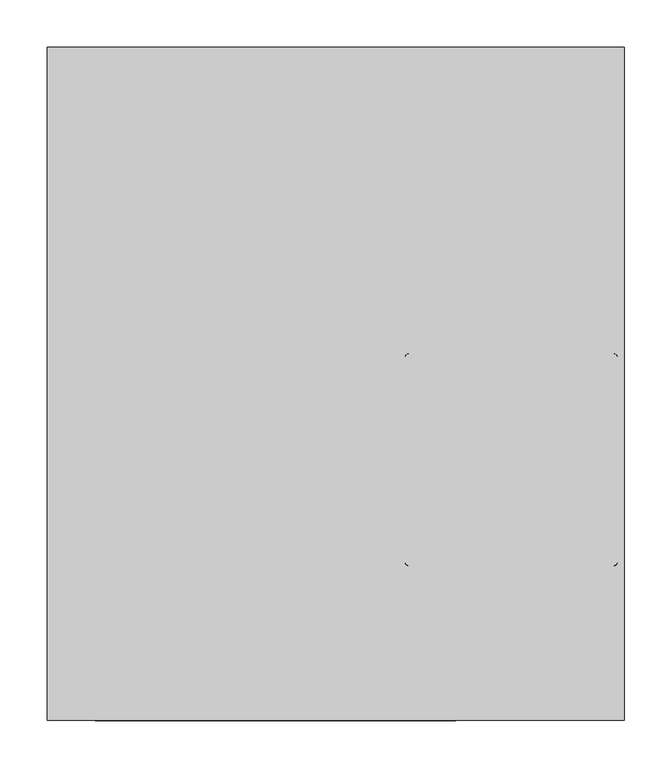
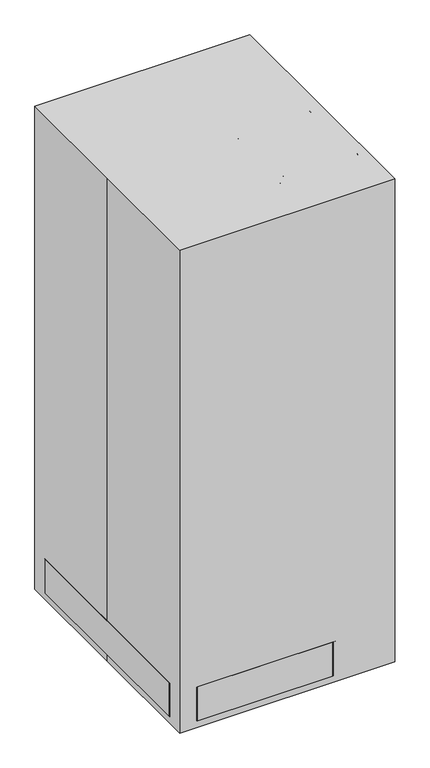
"""IFC4 building model written with IfcOpenShell, lengths in millimetres: proxy geometry, M1715 - Hemodialysis Unit, Hollow Fiber or Plate : M1715 - Hemodialysis Unit, Hollow Fiber or Plate."""

from ifc_helpers import new_model, si_unit, point, frame, frame_2d, origin, origin_with_axes, place, context, project, spatial, polyline, circle_curve, ellipse_curve, trimmed, segment, composite_curve, outline, extrude, source, transform, mapped, element, save
from ifc_brep_helpers import plane_surface, cylinder_surface, revolved_surface, advanced_brep


def specialty_equipment_02c0782f(model_context):
    return source(origin(), model_context, "Body", "SolidModel", [
        extrude(outline(polyline([(12.8462109, 171.45), (12.8462109, 165.1), (-152.2537891, 165.1), (-152.2537891, 171.45), (12.8462109, 171.45)])), frame((0.0, 0.0, 953.8161521), z_axis=(0.0, 0.0, 1.0), x_axis=(1.0, 0.0, 0.0)), (0.0, 0.0, 1.0), 127.0),
        extrude(outline(polyline([(152.4, -101.6), (209.55, -101.6), (209.55, -55.2125267), (152.4, -55.2125267), (152.4, -42.5125267), (222.25, -42.5125267), (222.25, -114.3), (152.4, -114.3), (152.4, -101.6)])), frame((0.0, 0.0, 812.8), z_axis=(0.0, 0.0, 1.0), x_axis=(1.0, 0.0, 0.0)), (0.0, 0.0, 1.0), 25.4),
        extrude(outline(polyline([(928.4161521, 38.2462109), (1106.2161521, 38.2462109), (1106.2161521, -177.6537891), (928.4161521, -177.6537891), (928.4161521, 38.2462109)]), holes=[polyline([(1080.8161521, -152.2537891), (1080.8161521, 12.8462109), (953.8161521, 12.8462109), (953.8161521, -152.2537891), (1080.8161521, -152.2537891)])]), frame((0.0, 165.1, 0.0), z_axis=(0.0, 1.0, 0.0), x_axis=(0.0, 0.0, 1.0)), (0.0, 0.0, 1.0), 6.35),
        extrude(outline(polyline([(421.0082083, 215.9), (421.0082083, 152.4), (281.3082083, 152.4), (344.8082083, 215.9), (421.0082083, 215.9)])), frame((0.0, -117.475, 0.0), z_axis=(0.0, 1.0, 0.0), x_axis=(0.0, 0.0, 1.0)), (0.0, 0.0, 1.0), 76.2),
        extrude(outline(composite_curve([segment(trimmed(circle_curve(frame_2d((555.4484832, 75.5254157)), 19.05), [point((555.4484832, 56.4754157))], [point((555.4484832, 94.5754157))], False, "CARTESIAN"), True, "CONTINUOUS"), segment(trimmed(circle_curve(frame_2d((555.4484832, 75.5254157)), 19.05), [point((555.4484832, 94.5754157))], [point((555.4484832, 56.4754157))], False, "CARTESIAN"), True, "CONTINUOUS")], self_intersect=False)), frame((0.0, 165.1, 0.0), z_axis=(0.0, 1.0, 0.0), x_axis=(0.0, 0.0, 1.0)), (0.0, 0.0, 1.0), 38.1),
        extrude(outline(composite_curve([segment(trimmed(circle_curve(frame_2d((555.4484832, 15.2004157)), 19.05), [point((555.4484832, -3.8495843))], [point((555.4484832, 34.2504157))], False, "CARTESIAN"), True, "CONTINUOUS"), segment(trimmed(circle_curve(frame_2d((555.4484832, 15.2004157)), 19.05), [point((555.4484832, 34.2504157))], [point((555.4484832, -3.8495843))], False, "CARTESIAN"), True, "CONTINUOUS")], self_intersect=False)), frame((0.0, 165.1, 0.0), z_axis=(0.0, 1.0, 0.0), x_axis=(0.0, 0.0, 1.0)), (0.0, 0.0, 1.0), 38.1),
        extrude(outline(composite_curve([segment(trimmed(circle_curve(frame_2d((555.4484832, -48.2995843)), 19.05), [point((555.4484832, -67.3495843))], [point((555.4484832, -29.2495843))], False, "CARTESIAN"), True, "CONTINUOUS"), segment(trimmed(circle_curve(frame_2d((555.4484832, -48.2995843)), 19.05), [point((555.4484832, -29.2495843))], [point((555.4484832, -67.3495843))], False, "CARTESIAN"), True, "CONTINUOUS")], self_intersect=False)), frame((0.0, 165.1, 0.0), z_axis=(0.0, 1.0, 0.0), x_axis=(0.0, 0.0, 1.0)), (0.0, 0.0, 1.0), 38.1),
        extrude(outline(composite_curve([segment(trimmed(circle_curve(frame_2d((555.4470563, -115.3669113)), 19.05), [point((555.4470563, -134.4169113))], [point((555.4470563, -96.3169113))], False, "CARTESIAN"), True, "CONTINUOUS"), segment(trimmed(circle_curve(frame_2d((555.4470563, -115.3669113)), 19.05), [point((555.4470563, -96.3169113))], [point((555.4470563, -134.4169113))], False, "CARTESIAN"), True, "CONTINUOUS")], self_intersect=False)), frame((0.0, 165.1, 0.0), z_axis=(0.0, 1.0, 0.0), x_axis=(0.0, 0.0, 1.0)), (0.0, 0.0, 1.0), 38.1),
        extrude(outline(polyline([(136.6593258, 165.1), (136.6593258, 127.0), (60.4593258, 127.0), (60.4593258, 165.1), (136.6593258, 165.1)])), frame((0.0, 0.0, 792.3608314), z_axis=(0.0, 0.0, 1.0), x_axis=(1.0, 0.0, 0.0)), (0.0, 0.0, 1.0), 38.1),
        extrude(outline(polyline([(36.523558, 165.1), (36.523558, 127.0), (-39.676442, 127.0), (-39.676442, 165.1), (36.523558, 165.1)])), frame((0.0, 0.0, 716.1608314), z_axis=(0.0, 0.0, 1.0), x_axis=(1.0, 0.0, 0.0)), (0.0, 0.0, 1.0), 114.3),
        extrude(outline(polyline([(-66.5406742, 165.1), (-66.5406742, 127.0), (-142.7406742, 127.0), (-142.7406742, 165.1), (-66.5406742, 165.1)])), frame((0.0, 0.0, 716.1608314), z_axis=(0.0, 0.0, 1.0), x_axis=(1.0, 0.0, 0.0)), (0.0, 0.0, 1.0), 114.3),
        extrude(outline(polyline([(-180.8406742, 165.1), (-180.8406742, 127.0), (-257.0406742, 127.0), (-257.0406742, 165.1), (-180.8406742, 165.1)])), frame((0.0, 0.0, 716.1608314), z_axis=(0.0, 0.0, 1.0), x_axis=(1.0, 0.0, 0.0)), (0.0, 0.0, 1.0), 38.1),
        extrude(outline(polyline([(-180.8406742, 165.1), (-180.8406742, 127.0), (-257.0406742, 127.0), (-257.0406742, 165.1), (-180.8406742, 165.1)])), frame((0.0, 0.0, 792.3608314), z_axis=(0.0, 0.0, 1.0), x_axis=(1.0, 0.0, 0.0)), (0.0, 0.0, 1.0), 38.1),
        extrude(outline(polyline([(140.5982906, 165.1), (140.5982906, 127.0), (-265.8017094, 127.0), (-265.8017094, 165.1), (140.5982906, 165.1)])), frame((0.0, 0.0, 446.4082083), z_axis=(0.0, 0.0, 1.0), x_axis=(1.0, 0.0, 0.0)), (0.0, 0.0, 1.0), 219.3819435),
        extrude(outline(polyline([(140.5982906, 165.1), (140.5982906, 127.0), (-265.8017094, 127.0), (-265.8017094, 165.1), (140.5982906, 165.1)])), frame((0.0, 0.0, 903.6082083), z_axis=(0.0, 0.0, 1.0), x_axis=(1.0, 0.0, 0.0)), (0.0, 0.0, 1.0), 219.3819435),
        extrude(outline(polyline([(140.5982906, 165.1), (140.5982906, 127.0), (-265.8017094, 127.0), (-265.8017094, 165.1), (140.5982906, 165.1)])), frame((0.0, 0.0, 132.3901517), z_axis=(0.0, 0.0, 1.0), x_axis=(1.0, 0.0, 0.0)), (0.0, 0.0, 1.0), 304.8),
        extrude(outline(polyline([(152.4, 127.0), (152.4, -279.4), (-279.4, -279.4), (-279.4, 127.0), (152.4, 127.0)])), frame((0.0, 0.0, 120.65), z_axis=(0.0, 0.0, 1.0), x_axis=(1.0, 0.0, 0.0)), (0.0, 0.0, 1.0), 1016.0),
        extrude(outline(composite_curve([segment(trimmed(circle_curve(frame_2d((185.3788167, -80.0577972)), 6.35), [point((179.0288167, -80.0577972))], [point((191.7288167, -80.0577972))], False, "CARTESIAN"), True, "CONTINUOUS"), segment(trimmed(circle_curve(frame_2d((185.3788167, -80.0577972)), 6.35), [point((191.7288167, -80.0577972))], [point((179.0288167, -80.0577972))], False, "CARTESIAN"), True, "CONTINUOUS")], self_intersect=False)), frame((0.0, 0.0, 1041.4), z_axis=(0.0, 0.0, 1.0), x_axis=(1.0, 0.0, 0.0)), (0.0, 0.0, 1.0), 388.3436057),
        advanced_brep(
        [(268.446484, -163.1254645, 1421.2516191), (264.5038206, -159.1828011, 1413.5291561), (276.9334178, -171.6123983, 1400.8374235), (280.8760812, -175.5550617, 1408.5598865), (284.1616341, -178.8406146, 1432.4577724), (284.1616341, -178.8406146, 1422.9327724), (86.5959994, 18.7250201, 1432.4577724), (86.5959994, 18.7250201, 1422.9327724), (93.8242157, 11.4968038, 1400.8374235), (89.8815523, 15.4394673, 1408.5598865), (102.3111494, 3.0098701, 1421.2516191), (106.2538129, -0.9327933, 1413.5291561)],
        [
            (0, 1, circle_curve(frame((266.4751523, -161.1541328, 1417.3903876), z_axis=(-0.5732919666883985, 0.5732919666884023, 0.5853824748496423), x_axis=(-0.41392791755394504, 0.41392791755394626, -0.8107572744902805)), 4.7625)),
            (1, 0, circle_curve(frame((266.4751523, -161.1541328, 1417.3903876), z_axis=(-0.5732919666883985, 0.5732919666884023, 0.5853824748496423), x_axis=(-0.41392791755394504, 0.41392791755394626, -0.8107572744902805)), 4.7625)),
            (1, 2),
            (2, 3, circle_curve(frame((278.9047495, -173.58373, 1404.698655), z_axis=(-0.5732919666883985, 0.5732919666884023, 0.5853824748496423), x_axis=(-0.41392791755394504, 0.41392791755394626, -0.8107572744902805)), 4.7625)),
            (3, 0),
            (3, 2, circle_curve(frame((278.9047495, -173.58373, 1404.698655), z_axis=(-0.5732919666883985, 0.5732919666884023, 0.5853824748496423), x_axis=(-0.41392791755394504, 0.41392791755394626, -0.8107572744902805)), 4.7625)),
            (4, 5, circle_curve(frame((284.1616341, -178.8406146, 1427.6952724), z_axis=(0.7071067811865466, -0.7071067811865487, 0.0), x_axis=(0.0, 0.0, 1.0)), 4.7625)),
            (5, 3, circle_curve(frame((284.1616341, -178.8406146, 1414.9952724), z_axis=(0.7071067811865489, 0.7071067811865462, 0.0), x_axis=(-0.413927917553943, 0.4139279175539444, -0.8107572744902825)), 7.9375)),
            (2, 4, circle_curve(frame((284.1616341, -178.8406146, 1414.9952724), z_axis=(-0.7071067811865489, -0.7071067811865462, 0.0), x_axis=(-0.413927917553943, 0.4139279175539444, -0.8107572744902825)), 17.4625)),
            (5, 4, circle_curve(frame((284.1616341, -178.8406146, 1427.6952724), z_axis=(0.7071067811865465, -0.7071067811865486, 0.0), x_axis=(0.0, 0.0, 1.0)), 4.7625)),
            (4, 6),
            (6, 7, circle_curve(frame((86.5959994, 18.7250201, 1427.6952724), z_axis=(0.7071067811865464, -0.7071067811865488, 0.0), x_axis=(0.0, 0.0, 1.0)), 4.7625)),
            (7, 5),
            (7, 6, circle_curve(frame((86.5959994, 18.7250201, 1427.6952724), z_axis=(0.7071067811865464, -0.7071067811865488, 0.0), x_axis=(0.0, 0.0, 1.0)), 4.7625)),
            (8, 9, circle_curve(frame((91.852884, 13.4681356, 1404.698655), z_axis=(-0.5732919666879008, 0.5732919666879034, -0.5853824748506183), x_axis=(0.4139279175546348, -0.41392791755463687, -0.8107572744895757)), 4.7625)),
            (9, 7, circle_curve(frame((86.5959994, 18.7250201, 1414.9952724), z_axis=(0.7071067811865489, 0.7071067811865462, 0.0), x_axis=(0.0, 0.0, 1.0)), 7.9375)),
            (6, 8, circle_curve(frame((86.5959994, 18.7250201, 1414.9952724), z_axis=(-0.7071067811865489, -0.7071067811865462, 0.0), x_axis=(0.0, 0.0, 1.0)), 17.4625)),
            (9, 8, circle_curve(frame((91.852884, 13.4681356, 1404.698655), z_axis=(-0.5732919666886381, 0.5732919666886407, -0.5853824748491742), x_axis=(0.41392791755361363, -0.4139279175536157, -0.8107572744906184)), 4.7625)),
            (10, 11, circle_curve(frame((104.2824812, 1.0385384, 1417.3903876), z_axis=(0.5732919666881265, -0.57329196668813, 0.5853824748501754), x_axis=(0.4139279175543215, -0.4139279175543237, -0.8107572744898957)), 4.7625)),
            (11, 10, circle_curve(frame((104.2824812, 1.0385384, 1417.3903876), z_axis=(0.5732919666881265, -0.57329196668813, 0.5853824748501754), x_axis=(0.4139279175543215, -0.4139279175543237, -0.8107572744898957)), 4.7625)),
            (8, 11),
            (10, 9),
        ],
        [
            plane_surface(frame((455.0605309, 27.4312457, 1417.3903876), z_axis=(-0.5732919666883985, 0.5732919666884023, 0.5853824748496423), x_axis=(-0.7071067811865496, -0.7071067811865456, 0.0))),
            cylinder_surface(frame((266.4751523, -161.1541328, 1417.3903876), z_axis=(-0.5732919666883985, 0.5732919666884023, 0.5853824748496423), x_axis=(-0.41392791755394504, 0.41392791755394626, -0.8107572744902805)), 4.7625),
            revolved_surface(trimmed(ellipse_curve(frame((278.9047495, -173.58373, 1404.698655), z_axis=(0.5732919666884007, -0.5732919666884032, -0.5853824748496393), x_axis=(-0.4139279175539432, 0.413927917553944, -0.8107572744902826)), 4.7625, 4.7625), [point((280.8760812, -175.5550617, 1408.5598865))], [point((276.9334178, -171.6123983, 1400.8374235))], True, "CARTESIAN"), (472.7470126, 9.744764, 1414.9952724), (0.7071067811865489, 0.7071067811865462, 0.0)),
            revolved_surface(trimmed(ellipse_curve(frame((278.9047495, -173.58373, 1404.698655), z_axis=(0.5732919666884007, -0.5732919666884032, -0.5853824748496393), x_axis=(-0.4139279175539432, 0.413927917553944, -0.8107572744902826)), 4.7625, 4.7625), [point((276.9334178, -171.6123983, 1400.8374235))], [point((280.8760812, -175.5550617, 1408.5598865))], True, "CARTESIAN"), (472.7470126, 9.744764, 1414.9952724), (0.7071067811865489, 0.7071067811865462, 0.0)),
            cylinder_surface(frame((284.1616341, -178.8406146, 1427.6952724), z_axis=(0.7071067811865464, -0.7071067811865488, 0.0), x_axis=(0.0, 0.0, 1.0)), 4.7625),
            revolved_surface(trimmed(ellipse_curve(frame((86.5959994, 18.7250201, 1427.6952724), z_axis=(-0.7071067811865465, 0.7071067811865487, 0.0), x_axis=(0.0, 0.0, 1.0)), 4.7625, 4.7625), [point((86.5959994, 18.7250201, 1422.9327724))], [point((86.5959994, 18.7250201, 1432.4577724))], True, "CARTESIAN"), (275.181378, 207.3103986, 1414.9952724), (0.7071067811865489, 0.7071067811865462, 0.0)),
            revolved_surface(trimmed(ellipse_curve(frame((86.5959994, 18.7250201, 1427.6952724), z_axis=(-0.7071067811865465, 0.7071067811865487, 0.0), x_axis=(0.0, 0.0, 1.0)), 4.7625, 4.7625), [point((86.5959994, 18.7250201, 1432.4577724))], [point((86.5959994, 18.7250201, 1422.9327724))], True, "CARTESIAN"), (275.181378, 207.3103986, 1414.9952724), (0.7071067811865489, 0.7071067811865462, 0.0)),
            plane_surface(frame((292.8678597, 189.6239169, 1417.3903876), z_axis=(0.5732919666881265, -0.5732919666881301, 0.5853824748501755), x_axis=(-0.7071067811865495, -0.7071067811865457, 0.0))),
            cylinder_surface(frame((91.852884, 13.4681356, 1404.698655), z_axis=(-0.5732919666881267, 0.5732919666881301, -0.5853824748501755), x_axis=(0.4139279175543215, -0.4139279175543237, -0.8107572744898957)), 4.7625),
        ],
        [
            (0, [[1, 2]]),
            (1, [[3, 4, 5, -2]]),
            (1, [[-5, 6, -3, -1]]),
            (2, [[7, 8, -4, 9]]),
            (3, [[10, -9, -6, -8]]),
            (4, [[11, 12, 13, -7]]),
            (4, [[-13, 14, -11, -10]]),
            (5, [[15, 16, -12, 17]]),
            (6, [[18, -17, -14, -16]]),
            (7, [[19, 20]]),
            (8, [[21, -19, 22, -15]]),
            (8, [[-22, -20, -21, -18]]),
        ],
    ),
        advanced_brep(
        [(102.3111494, -163.1254645, 1421.2516191), (106.2538129, -159.1828011, 1413.5291561), (93.8242157, -171.6123983, 1400.8374235), (89.8815523, -175.5550617, 1408.5598865), (86.5959994, -178.8406146, 1432.4577724), (86.5959994, -178.8406146, 1422.9327724), (284.1616341, 18.7250201, 1432.4577724), (284.1616341, 18.7250201, 1422.9327724), (276.9334178, 11.4968038, 1400.8374235), (280.8760812, 15.4394673, 1408.5598865), (268.446484, 3.0098701, 1421.2516191), (264.5038206, -0.9327933, 1413.5291561)],
        [
            (0, 1, circle_curve(frame((104.2824812, -161.1541328, 1417.3903876), z_axis=(0.5732919666884055, 0.5732919666884047, 0.5853824748496331), x_axis=(0.41392791755393954, 0.4139279175539388, -0.8107572744902871)), 4.7625)),
            (1, 0, circle_curve(frame((104.2824812, -161.1541328, 1417.3903876), z_axis=(0.5732919666884055, 0.5732919666884047, 0.5853824748496331), x_axis=(0.41392791755393954, 0.4139279175539388, -0.8107572744902871)), 4.7625)),
            (1, 2),
            (2, 3, circle_curve(frame((91.852884, -173.58373, 1404.698655), z_axis=(0.5732919666884055, 0.5732919666884047, 0.5853824748496331), x_axis=(0.41392791755393954, 0.4139279175539388, -0.8107572744902871)), 4.7625)),
            (3, 0),
            (3, 2, circle_curve(frame((91.852884, -173.58373, 1404.698655), z_axis=(0.5732919666884055, 0.5732919666884047, 0.5853824748496331), x_axis=(0.41392791755393954, 0.4139279175539388, -0.8107572744902871)), 4.7625)),
            (4, 5, circle_curve(frame((86.5959994, -178.8406146, 1427.6952724), z_axis=(-0.7071067811865482, -0.7071067811865468, 0.0), x_axis=(0.0, 0.0, 1.0)), 4.7625)),
            (5, 3, circle_curve(frame((86.5959994, -178.8406146, 1414.9952724), z_axis=(0.7071067811865469, -0.7071067811865482, 0.0), x_axis=(0.41392791755393793, 0.41392791755393726, -0.8107572744902887)), 7.9375)),
            (2, 4, circle_curve(frame((86.5959994, -178.8406146, 1414.9952724), z_axis=(-0.7071067811865469, 0.7071067811865482, 0.0), x_axis=(0.41392791755393793, 0.41392791755393726, -0.8107572744902887)), 17.4625)),
            (5, 4, circle_curve(frame((86.5959994, -178.8406146, 1427.6952724), z_axis=(-0.7071067811865482, -0.7071067811865467, 0.0), x_axis=(0.0, 0.0, 1.0)), 4.7625)),
            (4, 6),
            (6, 7, circle_curve(frame((284.1616341, 18.7250201, 1427.6952724), z_axis=(-0.7071067811865485, -0.7071067811865468, 0.0), x_axis=(0.0, 0.0, 1.0)), 4.7625)),
            (7, 5),
            (7, 6, circle_curve(frame((284.1616341, 18.7250201, 1427.6952724), z_axis=(-0.7071067811865485, -0.7071067811865468, 0.0), x_axis=(0.0, 0.0, 1.0)), 4.7625)),
            (8, 9, circle_curve(frame((278.9047495, 13.4681356, 1404.698655), z_axis=(0.5732919666881393, 0.5732919666881384, -0.5853824748501546), x_axis=(-0.4139279175543083, -0.4139279175543076, -0.8107572744899105)), 4.7625)),
            (9, 7, circle_curve(frame((284.1616341, 18.7250201, 1414.9952724), z_axis=(0.7071067811865469, -0.7071067811865482, 0.0), x_axis=(0.0, 0.0, 1.0)), 7.9375)),
            (6, 8, circle_curve(frame((284.1616341, 18.7250201, 1414.9952724), z_axis=(-0.7071067811865469, 0.7071067811865482, 0.0), x_axis=(0.0, 0.0, 1.0)), 17.4625)),
            (9, 8, circle_curve(frame((278.9047495, 13.4681356, 1404.698655), z_axis=(0.5732919666881443, 0.5732919666881434, -0.5853824748501448), x_axis=(-0.4139279175543014, -0.4139279175543007, -0.8107572744899176)), 4.7625)),
            (10, 11, circle_curve(frame((266.4751523, 1.0385384, 1417.3903876), z_axis=(-0.573291966688132, -0.5732919666881312, 0.5853824748501687), x_axis=(-0.4139279175543183, -0.4139279175543175, -0.8107572744899004)), 4.7625)),
            (11, 10, circle_curve(frame((266.4751523, 1.0385384, 1417.3903876), z_axis=(-0.573291966688132, -0.5732919666881312, 0.5853824748501687), x_axis=(-0.4139279175543183, -0.4139279175543175, -0.8107572744899004)), 4.7625)),
            (8, 11),
            (10, 9),
        ],
        [
            plane_surface(frame((256.9468352, -313.8184869, 1417.3903876), z_axis=(0.5732919666884055, 0.5732919666884047, 0.5853824748496331), x_axis=(-0.7071067811865469, 0.7071067811865481, 0.0))),
            cylinder_surface(frame((104.2824812, -161.1541328, 1417.3903876), z_axis=(0.5732919666884055, 0.5732919666884047, 0.5853824748496331), x_axis=(0.41392791755393954, 0.4139279175539388, -0.8107572744902871)), 4.7625),
            revolved_surface(trimmed(ellipse_curve(frame((91.852884, -173.58373, 1404.698655), z_axis=(-0.5732919666884068, -0.5732919666884059, -0.5853824748496308), x_axis=(0.4139279175539379, 0.4139279175539371, -0.8107572744902888)), 4.7625, 4.7625), [point((89.8815523, -175.5550617, 1408.5598865))], [point((93.8242157, -171.6123983, 1400.8374235))], True, "CARTESIAN"), (239.2603535, -331.5049686, 1414.9952724), (0.7071067811865469, -0.7071067811865482, 0.0)),
            revolved_surface(trimmed(ellipse_curve(frame((91.852884, -173.58373, 1404.698655), z_axis=(-0.5732919666884068, -0.5732919666884059, -0.5853824748496308), x_axis=(0.4139279175539379, 0.4139279175539371, -0.8107572744902888)), 4.7625, 4.7625), [point((93.8242157, -171.6123983, 1400.8374235))], [point((89.8815523, -175.5550617, 1408.5598865))], True, "CARTESIAN"), (239.2603535, -331.5049686, 1414.9952724), (0.7071067811865469, -0.7071067811865482, 0.0)),
            cylinder_surface(frame((86.5959994, -178.8406146, 1427.6952724), z_axis=(-0.7071067811865485, -0.7071067811865468, 0.0), x_axis=(0.0, 0.0, 1.0)), 4.7625),
            revolved_surface(trimmed(ellipse_curve(frame((284.1616341, 18.7250201, 1427.6952724), z_axis=(0.7071067811865483, 0.7071067811865468, 0.0), x_axis=(0.0, 0.0, 1.0)), 4.7625, 4.7625), [point((284.1616341, 18.7250201, 1422.9327724))], [point((284.1616341, 18.7250201, 1432.4577724))], True, "CARTESIAN"), (436.8259881, -133.939334, 1414.9952724), (0.7071067811865469, -0.7071067811865482, 0.0)),
            revolved_surface(trimmed(ellipse_curve(frame((284.1616341, 18.7250201, 1427.6952724), z_axis=(0.7071067811865483, 0.7071067811865468, 0.0), x_axis=(0.0, 0.0, 1.0)), 4.7625, 4.7625), [point((284.1616341, 18.7250201, 1432.4577724))], [point((284.1616341, 18.7250201, 1422.9327724))], True, "CARTESIAN"), (436.8259881, -133.939334, 1414.9952724), (0.7071067811865469, -0.7071067811865482, 0.0)),
            plane_surface(frame((419.1395064, -151.6258157, 1417.3903876), z_axis=(-0.5732919666881322, -0.5732919666881313, 0.5853824748501685), x_axis=(-0.707106781186547, 0.7071067811865481, 0.0))),
            cylinder_surface(frame((278.9047495, 13.4681356, 1404.698655), z_axis=(0.5732919666881321, 0.5732919666881313, -0.5853824748501688), x_axis=(-0.4139279175543183, -0.4139279175543175, -0.8107572744899004)), 4.7625),
        ],
        [
            (0, [[1, 2]]),
            (1, [[3, 4, 5, -2]]),
            (1, [[-5, 6, -3, -1]]),
            (2, [[7, 8, -4, 9]]),
            (3, [[10, -9, -6, -8]]),
            (4, [[11, 12, 13, -7]]),
            (4, [[-13, 14, -11, -10]]),
            (5, [[15, 16, -12, 17]]),
            (6, [[18, -17, -14, -16]]),
            (7, [[19, 20]]),
            (8, [[21, -19, 22, -15]]),
            (8, [[-22, -20, -21, -18]]),
        ],
    ),
        extrude(outline(composite_curve([segment(trimmed(circle_curve(frame_2d((185.3788167, -80.0577972)), 12.7), [point((172.6788167, -80.0577972))], [point((198.0788167, -80.0577972))], False, "CARTESIAN"), True, "CONTINUOUS"), segment(trimmed(circle_curve(frame_2d((185.3788167, -80.0577972)), 12.7), [point((198.0788167, -80.0577972))], [point((172.6788167, -80.0577972))], False, "CARTESIAN"), True, "CONTINUOUS")], self_intersect=False)), frame((0.0, 0.0, 421.0082083), z_axis=(0.0, 0.0, 1.0), x_axis=(1.0, 0.0, 0.0)), (0.0, 0.0, 1.0), 620.3917917),
        extrude(outline(composite_curve([segment(polyline([(127.0, -355.6), (-254.0, -355.6)]), True, "CONTINUOUS"), segment(trimmed(circle_curve(frame_2d((-254.0, -304.8)), 50.8), [point((-254.0, -355.6))], [point((-304.8, -304.8))], False, "CARTESIAN"), True, "CONTINUOUS"), segment(polyline([(-304.8, -304.8), (-304.8, 304.8)]), True, "CONTINUOUS"), segment(trimmed(circle_curve(frame_2d((-254.0, 304.8)), 50.8), [point((-304.8, 304.8))], [point((-254.0, 355.6))], False, "CARTESIAN"), True, "CONTINUOUS"), segment(polyline([(-254.0, 355.6), (127.0, 355.6)]), True, "CONTINUOUS"), segment(trimmed(circle_curve(frame_2d((127.0, 304.8)), 50.8), [point((127.0, 355.6))], [point((177.8, 304.8))], False, "CARTESIAN"), True, "CONTINUOUS"), segment(polyline([(177.8, 304.8), (177.8, -304.8)]), True, "CONTINUOUS"), segment(trimmed(circle_curve(frame_2d((127.0, -304.8)), 50.8), [point((177.8, -304.8))], [point((127.0, -355.6))], False, "CARTESIAN"), True, "CONTINUOUS")], self_intersect=False)), frame((0.0, 0.0, 19.05), z_axis=(0.0, 0.0, 1.0), x_axis=(1.0, 0.0, 0.0)), (0.0, 0.0, 1.0), 101.6),
        extrude(outline(composite_curve([segment(trimmed(circle_curve(frame_2d((126.5819236, 288.1244095)), 38.1), [point((88.4819236, 288.1244095))], [point((164.6819236, 288.1244095))], False, "CARTESIAN"), True, "CONTINUOUS"), segment(trimmed(circle_curve(frame_2d((126.5819236, 288.1244095)), 38.1), [point((164.6819236, 288.1244095))], [point((88.4819236, 288.1244095))], False, "CARTESIAN"), True, "CONTINUOUS")], self_intersect=False)), origin_with_axes(), (0.0, 0.0, 1.0), 19.05),
        extrude(outline(composite_curve([segment(trimmed(circle_curve(frame_2d((126.5819236, -289.7255905)), 38.1), [point((88.4819236, -289.7255905))], [point((164.6819236, -289.7255905))], False, "CARTESIAN"), True, "CONTINUOUS"), segment(trimmed(circle_curve(frame_2d((126.5819236, -289.7255905)), 38.1), [point((164.6819236, -289.7255905))], [point((88.4819236, -289.7255905))], False, "CARTESIAN"), True, "CONTINUOUS")], self_intersect=False)), origin_with_axes(), (0.0, 0.0, 1.0), 19.05),
        extrude(outline(composite_curve([segment(trimmed(circle_curve(frame_2d((-248.0680764, 288.1244095)), 38.1), [point((-286.1680764, 288.1244095))], [point((-209.9680764, 288.1244095))], False, "CARTESIAN"), True, "CONTINUOUS"), segment(trimmed(circle_curve(frame_2d((-248.0680764, 288.1244095)), 38.1), [point((-209.9680764, 288.1244095))], [point((-286.1680764, 288.1244095))], False, "CARTESIAN"), True, "CONTINUOUS")], self_intersect=False)), origin_with_axes(), (0.0, 0.0, 1.0), 19.05),
        extrude(outline(composite_curve([segment(trimmed(circle_curve(frame_2d((-248.0680764, -289.7255905)), 38.1), [point((-286.1680764, -289.7255905))], [point((-209.9680764, -289.7255905))], False, "CARTESIAN"), True, "CONTINUOUS"), segment(trimmed(circle_curve(frame_2d((-248.0680764, -289.7255905)), 38.1), [point((-209.9680764, -289.7255905))], [point((-286.1680764, -289.7255905))], False, "CARTESIAN"), True, "CONTINUOUS")], self_intersect=False)), origin_with_axes(), (0.0, 0.0, 1.0), 19.05),
        extrude(outline(polyline([(-304.8, -355.6), (-304.8, 0.0), (-304.8, 355.6), (304.8, 355.6), (304.8, -355.6), (-304.8, -355.6)])), origin_with_axes(), (0.0, 0.0, 1.0), 1447.8),
    ])


if __name__ == "__main__":
    model = new_model("IFC4")
    model_context = context("Model", 3, world=origin())
    ifc_project = project(units=[si_unit("LENGTHUNIT", "METRE", prefix="MILLI")], contexts=[model_context])
    site = spatial("IfcSite", under=ifc_project)
    building = spatial("IfcBuilding", under=site)
    placement = place(None, origin())
    specialty_equipment_shape = specialty_equipment_02c0782f(model_context)
    element("IfcBuildingElementProxy", 1, Name="M1715 - Hemodialysis Unit, Hollow Fiber or Plate : M1715 - Hemodialysis Unit, Hollow Fiber or Plate", ObjectType="M1715 - Hemodialysis Unit, Hollow Fiber or Plate : M1715 - Hemodialysis Unit, Hollow Fiber or Plate", at=placement, inside=building, context=model_context, shape_type="MappedRepresentation", body=[
        mapped(specialty_equipment_shape, transform((0.0, 0.0, 0.0), x_axis=(1.0, 0.0, 0.0), y_axis=(0.0, 1.0, 0.0), z_axis=(0.0, 0.0, 1.0))),
    ])
    save(model, "model.ifc")

# Revit data of these elements
# Project information
#   Room Abbreviation = "RDC01"
#   Room Description = "Renal Dialysis, Airborne Infection Isolation (RDC01)"
#   Sheets - Total = "5"
#   Project Issue Date = "Issue Date"
#   Project Status = "Project Status"
#   Client Name = "Owner"
#   Project Address = "Enter address here"
#   Project Name = "Project Name"
#   Project Number = "Project Number"
#   Publication Date = "1-Feb-16"
# Type "M1715 - Hemodialysis Unit, Hollow Fiber or Plate : M1715 - Hemodialysis Unit, Hollow Fiber or Plate"
#   Watts2 = "0"
#   Watts1 = "1440"
#   Unit_Issue = "EA"
#   UTIL_6_Misc = "-"
#   UTIL_5_NonMedGas = "-"
#   UTIL_4_MiscGas = "-"
#   UTIL_3_MedGas = "-"
#   UTIL_2_Elec = "A"
#   UTIL_1_WaterDrain = "E"
#   Nomenclature = "Hemodialysis Unit, Hollow Fiber or Plate"
#   NSN = "6515"
#   Location [instance default] = ""
#   JSN = "M1715"
#   Fund_Source_VA = "-"
#   Fund_Source_Navy = "-"
#   Fund_Source_Army = "-"
#   Fund_Source_AF = "-"
#   ELEC_Volts2 = "0"
#   ELEC_Volts1 = "120"
#   ELEC_Phase2 = "0"
#   ELEC_Phase1 = "1"
#   ELEC_HertzSwitch = "0"
#   ELEC_HertzDependent = "-1"
#   ELEC_Hertz = "60"
#   ELEC_Amps2 = "0"
#   ELEC_Amps1 = "12"
#   DetailDescription = "Complete hemodialysis unit using either hollow fiber or plate type dialyzers. Unit is freestanding in a wheeled cabinet and include water connection, concentrate pickup pump, proportioner, conductivity monitor, dialysate heater, blood pump, heparin pump, arterial pressure monitor, venous pressure monitor, TMP monitor, air/foam detector, optical detector, blood leak detector, power failure alarm, and remote alarm contacts. Accommodates single needle, two pump procedures. Database information reflects mobile units which carry their own water purification systems. Predominately stationary units within a clinic area can operate from a central water purification system. Electrical circuit should include a ground fault interrupter. Variations of this equipment include versions for pediatric use and peritoneal dialysis (JSN M4860). Optional equipment includes blood pressure monitoring and a variety of waste handling options."
#   CAT_VA = "C"
#   CAT_Navy = "C"
#   CAT_IHS = "-"
#   CAT_Army = "C"
#   CAT_AF = "C"
#   BTUperhour = "0"
#   Weight_IP = 264
#   DIM_Width_IP = 2' - 0"
#   DIM_Height_IP = 4' - 9"
#   DIM_Depth_IP = 2' - 4"
#   finish [instance default] = none
# Element 1 (IfcBuildingElementProxy, "M1715 - Hemodialysis Unit, Hollow Fiber or Plate : M1715 - Hemodialysis Unit, Hollow Fiber or Plate")
#   Materials on its faces: "EquipSpace", "Glass"
# Materials
#   "EquipSpace": class "Unassigned", colour RGB 221 217 195, transparency 0.5
#   "Glass": class "Glass", colour RGB 0 128 192, transparency 0.75
